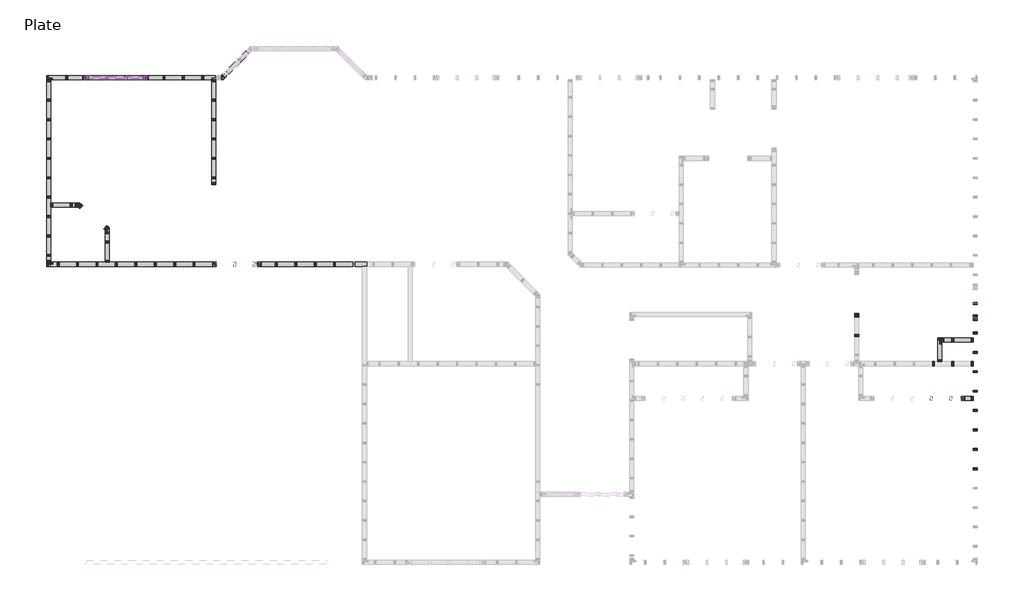
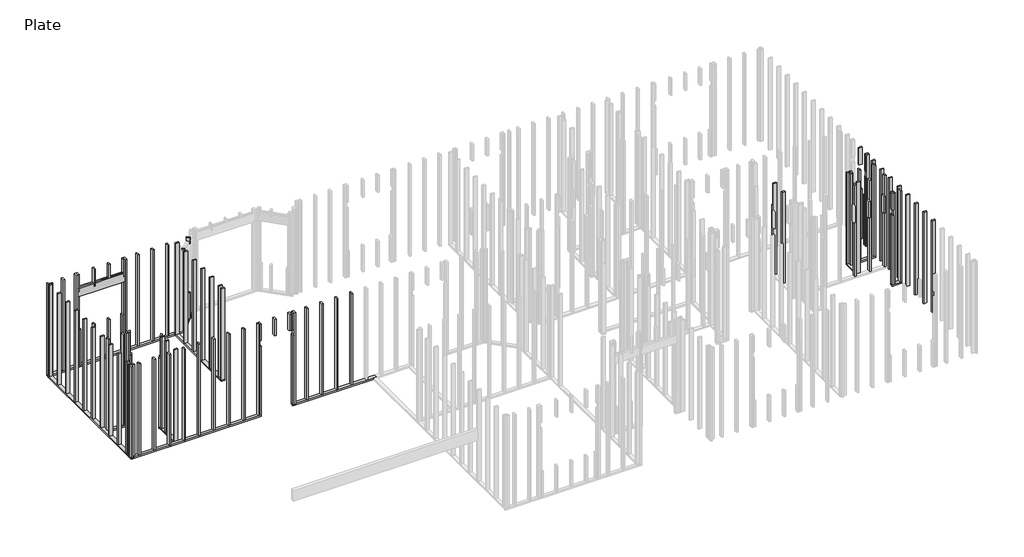
# One storey, part 3 of 5: 104 columns, 15 beams.
"""IFC4 building model written with IfcOpenShell, lengths in millimetres."""

import ifcopenshell
import ifcopenshell.guid

model = None  # the IFC model being written
_history = None  # IfcOwnerHistory: only IFC2X3 demands one
_inside = {}  # id of a spatial element -> (the spatial element, [elements in it])
_under = {}  # id of a project, library or spatial element -> (it, [spatial elements below it])
_declared = {}  # id of a project -> (the project, [libraries it declares])
_typed = {}  # id of a type object -> (the type object, [elements of that type])
_made_of = {}  # id of a material, layer set ... -> (it, [elements and type objects made of it])


def new_model(schema):
    """Start an empty IFC model of exactly this schema.

    Asked for "IFC4X3", IfcOpenShell would pick the latest addendum, in which some entities
    have other attributes; the version numbers below select the first issue.
    IFC2X3 requires an IfcOwnerHistory on every rooted entity: one is made here for all.
    """
    global model, _history
    if schema == "IFC4X3":
        model = ifcopenshell.file(schema_version=(4, 3, 0, 0))
    else:
        model = ifcopenshell.file(schema=schema)
    _inside.clear()
    _under.clear()
    _declared.clear()
    _typed.clear()
    _made_of.clear()
    _history = None
    if model.schema == "IFC2X3":
        org = make("IfcOrganization", Name="unknown")
        user = make(
            "IfcPersonAndOrganization",
            ThePerson=make("IfcPerson", FamilyName="unknown"),
            TheOrganization=org,
        )
        app = make(
            "IfcApplication",
            ApplicationDeveloper=org,
            Version="unknown",
            ApplicationFullName="unknown",
            ApplicationIdentifier="unknown",
        )
        _history = make(
            "IfcOwnerHistory",
            OwningUser=user,
            OwningApplication=app,
            ChangeAction="ADDED",
            CreationDate=0,
        )
    return model


def make(cls, **values):
    """One entity of the class cls with the attributes given. An attribute that is None is left unset."""
    return model.create_entity(
        cls, **{name: value for name, value in values.items() if value is not None}
    )


def rooted(cls, **values):
    """An entity with a GlobalId (a new one), such as an element, a storey or a relation."""
    return make(cls, GlobalId=ifcopenshell.guid.new(), OwnerHistory=_history, **values)


def si_unit(unit_type, name, prefix=None):
    """IfcSIUnit, for example si_unit("LENGTHUNIT", "METRE", prefix="MILLI")."""
    return make("IfcSIUnit", UnitType=unit_type, Prefix=prefix, Name=name)


def assignment(units):
    """IfcUnitAssignment: the units of a project."""
    return None if units is None else make("IfcUnitAssignment", Units=units)


def point(xyz):
    """IfcCartesianPoint."""
    return None if xyz is None else make("IfcCartesianPoint", Coordinates=xyz)


def direction(xyz):
    """IfcDirection."""
    return None if xyz is None else make("IfcDirection", DirectionRatios=xyz)


def frame(location, z_axis=None, x_axis=None):
    """IfcAxis2Placement3D, a coordinate frame: its origin and axes. An axis left out is left unset."""
    return make(
        "IfcAxis2Placement3D",
        Location=point(location),
        Axis=direction(z_axis),
        RefDirection=direction(x_axis),
    )


def origin():
    """The frame at (0, 0, 0) with its axes left unset."""
    return frame((0.0, 0.0, 0.0))


def place(relative_to, where):
    """IfcLocalPlacement: puts the frame where relative to a parent placement (None: the world)."""
    return make(
        "IfcLocalPlacement", PlacementRelTo=relative_to, RelativePlacement=where
    )


def context(
    kind, dimensions, precision=None, world=None, true_north=None, identifier=None
):
    """IfcGeometricRepresentationContext, for example the 3D "Model" context."""
    return make(
        "IfcGeometricRepresentationContext",
        ContextIdentifier=identifier,
        ContextType=kind,
        CoordinateSpaceDimension=dimensions,
        Precision=precision,
        WorldCoordinateSystem=world,
        TrueNorth=true_north,
    )


def project(units=None, contexts=None):
    """IfcProject with its units and contexts."""
    return rooted(
        "IfcProject",
        Name="project",
        RepresentationContexts=contexts,
        UnitsInContext=assignment(units),
    )


def spatial(cls, under=None, at=None, **own):
    """A site, building, storey or space (cls), placed at a placement, below another one or the project."""
    s = rooted(cls, ObjectPlacement=at, **own)
    if under is not None:
        _under.setdefault(under.id(), (under, []))[1].append(s)
    return s


def polyline(points):
    """IfcPolyline through the points."""
    return make("IfcPolyline", Points=[point(p) for p in points])


def outline(outer, holes=None, kind="AREA"):
    """IfcArbitraryClosedProfileDef: a profile drawn as a closed curve; with holes, ...WithVoids."""
    if holes is None:
        return make("IfcArbitraryClosedProfileDef", ProfileType=kind, OuterCurve=outer)
    return make(
        "IfcArbitraryProfileDefWithVoids",
        ProfileType=kind,
        OuterCurve=outer,
        InnerCurves=holes,
    )


def extrude(swept, where, along, depth):
    """IfcExtrudedAreaSolid: the profile swept, set in the frame where, extruded along a direction by depth."""
    return make(
        "IfcExtrudedAreaSolid",
        SweptArea=swept,
        Position=where,
        ExtrudedDirection=direction(along),
        Depth=depth,
    )


def shape(context_of_items, identifier, shape_type, items):
    """IfcShapeRepresentation: the items that make up one representation, for example the "Body"."""
    return make(
        "IfcShapeRepresentation",
        ContextOfItems=context_of_items,
        RepresentationIdentifier=identifier,
        RepresentationType=shape_type,
        Items=items,
    )


def source(mapping_origin, context_of_items, identifier, shape_type, items):
    """IfcRepresentationMap: a shape defined once, which mapped items show again and again."""
    return make(
        "IfcRepresentationMap",
        MappingOrigin=mapping_origin,
        MappedRepresentation=shape(context_of_items, identifier, shape_type, items),
    )


def transform(
    local_origin,
    x_axis=None,
    y_axis=None,
    z_axis=None,
    scale=None,
    scale2=None,
    scale3=None,
    uniform=True,
):
    """IfcCartesianTransformationOperator3D, or its non-uniform kind. x_axis, y_axis, z_axis: its Axis1, 2, 3."""
    if uniform:
        return make(
            "IfcCartesianTransformationOperator3D",
            Axis1=direction(x_axis),
            Axis2=direction(y_axis),
            LocalOrigin=point(local_origin),
            Scale=scale,
            Axis3=direction(z_axis),
        )
    return make(
        "IfcCartesianTransformationOperator3DnonUniform",
        Axis1=direction(x_axis),
        Axis2=direction(y_axis),
        LocalOrigin=point(local_origin),
        Scale=scale,
        Axis3=direction(z_axis),
        Scale2=scale2,
        Scale3=scale3,
    )


def mapped(mapping_source, mapping_target):
    """IfcMappedItem: shows the shape of a source again, moved by a transform."""
    return make(
        "IfcMappedItem", MappingSource=mapping_source, MappingTarget=mapping_target
    )


def made_of(thing, what):
    """Note that an element or type object is made of a material, layer set ...; save() writes the relation."""
    if what is not None:
        _made_of.setdefault(what.id(), (what, []))[1].append(thing)
    return thing


def element(
    cls,
    number,
    at=None,
    inside=None,
    cuts=None,
    type_object=None,
    material=None,
    context=None,
    identifier="Body",
    shape_type=None,
    held_by="IfcProductDefinitionShape",
    body=None,
    shapes=None,
    **own,
):
    """One element of the class cls, such as IfcWall. Its Tag is "e" and its number.

    at: its placement. inside: the storey or other place that contains it. cuts: it is an
    opening in that element (IfcRelVoidsElement). A single representation is given by context,
    identifier, shape_type and body (its items); several are given by shapes. held_by: the class
    of the entity that holds the representations. save() writes the other relations.
    """
    e = rooted(cls, Tag="e%d" % number, ObjectPlacement=at, **own)
    if body is not None:
        shapes = [shape(context, identifier, shape_type, body)]
    if shapes is not None:
        e.Representation = make(held_by, Representations=shapes)
    if inside is not None:
        _inside.setdefault(inside.id(), (inside, []))[1].append(e)
    if cuts is not None:
        rooted(
            "IfcRelVoidsElement", RelatingBuildingElement=cuts, RelatedOpeningElement=e
        )
    if type_object is not None:
        _typed.setdefault(type_object.id(), (type_object, []))[1].append(e)
    return made_of(e, material)


def aggregate(whole, parts):
    """IfcRelAggregates: a whole, such as a stair, and the parts it consists of."""
    return rooted("IfcRelAggregates", RelatingObject=whole, RelatedObjects=parts)


def save(model, path):
    """Write the relations noted so far, then the file.

    IfcRelAggregates (storeys below a building ...), IfcRelContainedInSpatialStructure (elements
    in a storey), IfcRelDefinesByType, IfcRelAssociatesMaterial and IfcRelDeclares: one each for
    every whole, place, type object, material and project.
    """
    for whole, parts in _under.values():
        aggregate(whole, parts)
    for where, things in _inside.values():
        rooted(
            "IfcRelContainedInSpatialStructure",
            RelatedElements=things,
            RelatingStructure=where,
        )
    for kind, things in _typed.values():
        rooted("IfcRelDefinesByType", RelatedObjects=things, RelatingType=kind)
    for what, things in _made_of.values():
        rooted("IfcRelAssociatesMaterial", RelatedObjects=things, RelatingMaterial=what)
    for by, libraries in _declared.values():
        rooted("IfcRelDeclares", RelatingContext=by, RelatedDefinitions=libraries)
    model.write(path)


def dimension_lumber_2x10_header_exterior_8d927054(model_context):
    return source(origin(), model_context, "Body", "SweptSolid", [
        extrude(outline(polyline([(468.709375, 19.05), (468.709375, -19.05), (-826.690625, -19.05), (-826.690625, 19.05), (468.709375, 19.05)])), frame((0.0, 0.0, -117.475), z_axis=(0.0, 0.0, 1.0), x_axis=(1.0, 0.0, 0.0)), (0.0, 0.0, 1.0), 234.95),
    ])


def dimension_lumber_supporting_bottom_plate_fd513b8e(model_context):
    return source(origin(), model_context, "Body", "SweptSolid", [
        extrude(outline(polyline([(1118.39375, 44.45), (1118.39375, -44.45), (-1165.225, -44.45), (-1165.225, 44.45), (1118.39375, 44.45)])), frame((0.0, 0.0, -19.05), z_axis=(0.0, 0.0, 1.0), x_axis=(1.0, 0.0, 0.0)), (0.0, 0.0, 1.0), 38.1),
    ])


def dimension_lumber_supporting_bottom_plate_14fdda6b(model_context):
    return source(origin(), model_context, "Body", "SweptSolid", [
        extrude(outline(polyline([(1910.55625, 44.45), (1910.55625, -44.45), (-1999.45625, -44.45), (-1999.45625, 44.45), (1910.55625, 44.45)])), frame((0.0, 0.0, -19.05), z_axis=(0.0, 0.0, 1.0), x_axis=(1.0, 0.0, 0.0)), (0.0, 0.0, 1.0), 38.1),
    ])


def dimension_lumber_supporting_bottom_plate_770482cb(model_context):
    return source(origin(), model_context, "Body", "SweptSolid", [
        extrude(outline(polyline([(1708.546875, 44.45), (1708.546875, -44.45), (-1752.996875, -44.45), (-1752.996875, 44.45), (1708.546875, 44.45)])), frame((0.0, 0.0, -19.05), z_axis=(0.0, 0.0, 1.0), x_axis=(1.0, 0.0, 0.0)), (0.0, 0.0, 1.0), 38.1),
    ])


def dimension_lumber_supporting_bottom_plate_d1710e57(model_context):
    return source(origin(), model_context, "Body", "SweptSolid", [
        extrude(outline(polyline([(1739.2219145, 44.45), (1739.2219145, -44.45), (-454.81875, -44.45), (-454.81875, 44.45), (1739.2219145, 44.45)])), frame((0.0, 0.0, -19.05), z_axis=(0.0, 0.0, 1.0), x_axis=(1.0, 0.0, 0.0)), (0.0, 0.0, 1.0), 38.1),
    ])


def dimension_lumber_supporting_bottom_plate_47a8c852(model_context):
    return source(origin(), model_context, "Body", "SweptSolid", [
        extrude(outline(polyline([(292.0, 44.45), (292.0, -44.45), (-203.1, -44.45), (-203.1, 44.45), (292.0, 44.45)])), frame((0.0, 0.0, -19.05), z_axis=(0.0, 0.0, 1.0), x_axis=(1.0, 0.0, 0.0)), (0.0, 0.0, 1.0), 38.1),
    ])


def dimension_lumber_supporting_bottom_plate_e3733361(model_context):
    return source(origin(), model_context, "Body", "SweptSolid", [
        extrude(outline(polyline([(328.9051334, 44.45), (328.9051334, -44.45), (-328.9051334, -44.45), (-328.9051334, 44.45), (328.9051334, 44.45)])), frame((0.0, 0.0, -19.05), z_axis=(0.0, 0.0, 1.0), x_axis=(1.0, 0.0, 0.0)), (0.0, 0.0, 1.0), 38.1),
    ])


def dimension_lumber_supporting_bottom_plate_76e17ce6(model_context):
    return source(origin(), model_context, "Body", "SweptSolid", [
        extrude(outline(polyline([(146.8437503, 44.45), (146.8437503, -44.45), (-102.3937503, -44.45), (-102.3937503, 44.45), (146.8437503, 44.45)])), frame((0.0, 0.0, -19.05), z_axis=(0.0, 0.0, 1.0), x_axis=(1.0, 0.0, 0.0)), (0.0, 0.0, 1.0), 38.1),
    ])


def dimension_lumber_column_2x4_07183c39(model_context):
    return source(origin(), model_context, "Body", "SweptSolid", [
        extrude(outline(polyline([(19.05, 44.45), (19.05, -44.45), (-19.05, -44.45), (-19.05, 44.45), (19.05, 44.45)])), frame((0.0, 0.0, 56.35625), z_axis=(0.0, 0.0, 1.0), x_axis=(1.0, 0.0, 0.0)), (0.0, 0.0, 1.0), 2636.04375),
    ])


def dimension_lumber_column_2x4_f24b5bbb(model_context):
    return source(origin(), model_context, "Body", "SweptSolid", [
        extrude(outline(polyline([(19.05, -44.45), (-19.05, -44.45), (-19.05, 44.45), (19.05, 44.45), (19.05, -44.45)])), frame((0.0, 0.0, 56.35625), z_axis=(0.0, 0.0, 1.0), x_axis=(1.0, 0.0, 0.0)), (0.0, 0.0, 1.0), 2636.04375),
    ])


def dimension_lumber_column_2x4_1c0ee4a5(model_context):
    return source(origin(), model_context, "Body", "SweptSolid", [
        extrude(outline(polyline([(19.05, -44.45), (-19.05, -44.45), (-19.05, 44.45), (19.05, 44.45), (19.05, -44.45)])), frame((0.0, 0.0, 56.35625), z_axis=(0.0, 0.0, 1.0), x_axis=(1.0, 0.0, 0.0)), (0.0, 0.0, 1.0), 2331.24375),
    ])


def dimension_lumber_column_2x4_0f816ddf(model_context):
    return source(origin(), model_context, "Body", "SweptSolid", [
        extrude(outline(polyline([(19.05, 44.45), (19.05, -44.45), (-19.05, -44.45), (-19.05, 44.45), (19.05, 44.45)])), frame((0.0, 0.0, 56.35625), z_axis=(0.0, 0.0, 1.0), x_axis=(1.0, 0.0, 0.0)), (0.0, 0.0, 1.0), 1999.853125),
    ])


def dimension_lumber_column_2x4_c2f848da(model_context):
    return source(origin(), model_context, "Body", "SweptSolid", [
        extrude(outline(polyline([(19.05, 44.45), (19.05, -44.45), (-19.05, -44.45), (-19.05, 44.45), (19.05, 44.45)])), frame((0.0, 0.0, 2208.609375), z_axis=(0.0, 0.0, 1.0), x_axis=(1.0, 0.0, 0.0)), (0.0, 0.0, 1.0), 483.790625),
    ])


def dimension_lumber_column_2x4_1a929157(model_context):
    return source(origin(), model_context, "Body", "SweptSolid", [
        extrude(outline(polyline([(19.05, 44.45), (19.05, -44.45), (-19.05, -44.45), (-19.05, 44.45), (19.05, 44.45)])), frame((0.0, 0.0, 2208.609375), z_axis=(0.0, 0.0, 1.0), x_axis=(1.0, 0.0, 0.0)), (0.0, 0.0, 1.0), 178.990625),
    ])


def dimension_lumber_column_2x4_35883525(model_context):
    return source(origin(), model_context, "Body", "SweptSolid", [
        extrude(outline(polyline([(19.05, 44.45), (19.05, -44.45), (-19.05, -44.45), (-19.05, 44.45), (19.05, 44.45)])), frame((0.0, 0.0, 56.35625), z_axis=(0.0, 0.0, 1.0), x_axis=(1.0, 0.0, 0.0)), (0.0, 0.0, 1.0), 742.553125),
    ])


def dimension_lumber_column_2x4_e2d4624f(model_context):
    return source(origin(), model_context, "Body", "SweptSolid", [
        extrude(outline(polyline([(19.05, 44.45), (19.05, -44.45), (-19.05, -44.45), (-19.05, 44.45), (19.05, 44.45)])), frame((0.0, 0.0, 56.35625), z_axis=(0.0, 0.0, 1.0), x_axis=(1.0, 0.0, 0.0)), (0.0, 0.0, 1.0), 1047.353125),
    ])


def dimension_lumber_column_2x4_c4e013fe(model_context):
    return source(origin(), model_context, "Body", "SweptSolid", [
        extrude(outline(polyline([(19.05, 44.45), (19.05, -44.45), (-19.05, -44.45), (-19.05, 44.45), (19.05, 44.45)])), frame((0.0, 0.0, 56.35625), z_axis=(0.0, 0.0, 1.0), x_axis=(1.0, 0.0, 0.0)), (0.0, 0.0, 1.0), 1444.228125),
    ])


model = new_model("IFC4")

# Units and contexts
model_context = context("Model", 3, world=origin())
ifc_project = project(units=[si_unit("LENGTHUNIT", "METRE", prefix="MILLI")], contexts=[model_context])

# Site, building, storey
site = spatial("IfcSite", under=ifc_project)
building = spatial("IfcBuilding", under=site)
storey = spatial("IfcBuildingStorey", under=building, Name="Plate", Elevation=56.35625)

# Beams
placement = place(None, origin())
dimension_lumber_2x10_header_exterior_shape = dimension_lumber_2x10_header_exterior_8d927054(model_context)
element("IfcBeam", 1, ObjectType="Dimension Lumber : 2x10 Header Exterior", at=placement, inside=storey, context=model_context, shape_type="MappedRepresentation", body=[
    mapped(dimension_lumber_2x10_header_exterior_shape, transform((-4972.0933507, 4418.3834053, 2173.684375), x_axis=(-1.0, 0.0, 0.0), y_axis=(0.0, -1.0, 0.0), z_axis=(0.0, 0.0, 1.0))),
])
element("IfcBeam", 2, ObjectType="Dimension Lumber : 2x10 Header Exterior", at=placement, inside=storey, context=model_context, shape_type="MappedRepresentation", body=[
    mapped(dimension_lumber_2x10_header_exterior_shape, transform((-4972.0933507, 4469.1834053, 2173.684375), x_axis=(-1.0, 0.0, 0.0), y_axis=(0.0, -1.0, 0.0), z_axis=(0.0, 0.0, 1.0))),
])
element("IfcBeam", 3, ObjectType="Dimension Lumber : Supporting Bottom Plate", at=placement, inside=storey, context=model_context, shape_type="SweptSolid", body=[
    extrude(outline(polyline([(-2583.3027251, 4488.2334053), (-2546.4791394, 4399.3334053), (-6240.9027251, 4399.3334053), (-6240.9027251, 4488.2334053), (-2583.3027251, 4488.2334053)])), frame((0.0, 0.0, 18.25625), z_axis=(0.0, 0.0, 1.0), x_axis=(1.0, 0.0, 0.0)), (0.0, 0.0, 1.0), 38.1),
])
element("IfcBeam", 4, ObjectType="Dimension Lumber : Supporting Bottom Plate", at=placement, inside=storey, context=model_context, shape_type="SweptSolid", body=[
    extrude(outline(polyline([(-1973.7027251, 5097.8334053), (-1936.8791394, 5008.9334053), (-2546.4791394, 4399.3334053), (-2583.3027251, 4488.2334053), (-1973.7027251, 5097.8334053)])), frame((0.0, 0.0, 18.25625), z_axis=(0.0, 0.0, 1.0), x_axis=(1.0, 0.0, 0.0)), (0.0, 0.0, 1.0), 38.1),
])
element("IfcBeam", 5, ObjectType="Dimension Lumber : Supporting Bottom Plate", at=placement, inside=storey, context=model_context, shape_type="SweptSolid", body=[
    extrude(outline(polyline([(-5544.0627459, 1818.4935621), (-5576.4196998, 1729.5935621), (-6152.0027251, 1729.5935621), (-6152.0027251, 1818.4935621), (-5544.0627459, 1818.4935621)])), frame((0.0, 0.0, 18.25625), z_axis=(0.0, 0.0, 1.0), x_axis=(1.0, 0.0, 0.0)), (0.0, 0.0, 1.0), 38.1),
])
element("IfcBeam", 6, ObjectType="Dimension Lumber : Supporting Bottom Plate", at=placement, inside=storey, context=model_context, shape_type="SweptSolid", body=[
    extrude(outline(polyline([(-5485.6901594, 1769.5131462), (-5542.8339779, 1701.4117952), (-5576.4196998, 1729.5935621), (-5544.0627459, 1818.4935621), (-5485.6901594, 1769.5131462)])), frame((0.0, 0.0, 18.25625), z_axis=(0.0, 0.0, 1.0), x_axis=(1.0, 0.0, 0.0)), (0.0, 0.0, 1.0), 38.1),
])
element("IfcBeam", 7, ObjectType="Dimension Lumber : Supporting Bottom Plate", at=placement, inside=storey, context=model_context, shape_type="SweptSolid", body=[
    extrude(outline(polyline([(-5012.1263621, 1256.0952306), (-4923.2263621, 1297.5499814), (-4923.2263621, 578.2209053), (-5012.1263621, 578.2209053), (-5012.1263621, 1256.0952306)])), frame((0.0, 0.0, 18.25625), z_axis=(0.0, 0.0, 1.0), x_axis=(1.0, 0.0, 0.0)), (0.0, 0.0, 1.0), 38.1),
])
element("IfcBeam", 8, ObjectType="Dimension Lumber : Supporting Bottom Plate", at=placement, inside=storey, context=model_context, shape_type="SweptSolid", body=[
    extrude(outline(polyline([(-4923.2263621, 1297.5499814), (-5012.1263621, 1256.0952306), (-5038.762371, 1278.4454958), (-4981.6185525, 1346.5468468), (-4923.2263621, 1297.5499814)])), frame((0.0, 0.0, 18.25625), z_axis=(0.0, 0.0, 1.0), x_axis=(1.0, 0.0, 0.0)), (0.0, 0.0, 1.0), 38.1),
])
dimension_lumber_supporting_bottom_plate_shape = dimension_lumber_supporting_bottom_plate_fd513b8e(model_context)
element("IfcBeam", 9, ObjectType="Dimension Lumber : Supporting Bottom Plate", at=placement, inside=storey, context=model_context, shape_type="MappedRepresentation", body=[
    mapped(dimension_lumber_supporting_bottom_plate_shape, transform((-708.4652251, 533.7709053, 37.30625), x_axis=(-1.0, 0.0, 0.0), y_axis=(0.0, -1.0, 0.0), z_axis=(0.0, 0.0, 1.0))),
])
dimension_lumber_supporting_bottom_plate_2_shape = dimension_lumber_supporting_bottom_plate_14fdda6b(model_context)
element("IfcBeam", 10, ObjectType="Dimension Lumber : Supporting Bottom Plate", at=placement, inside=storey, context=model_context, shape_type="MappedRepresentation", body=[
    mapped(dimension_lumber_supporting_bottom_plate_2_shape, transform((-6196.4527251, 2488.7771553, 37.30625), x_axis=(0.0, 1.0, 0.0), y_axis=(-1.0, 0.0, 0.0), z_axis=(0.0, 0.0, 1.0))),
])
dimension_lumber_supporting_bottom_plate_3_shape = dimension_lumber_supporting_bottom_plate_770482cb(model_context)
element("IfcBeam", 11, ObjectType="Dimension Lumber : Supporting Bottom Plate", at=placement, inside=storey, context=model_context, shape_type="MappedRepresentation", body=[
    mapped(dimension_lumber_supporting_bottom_plate_3_shape, transform((-4443.4558501, 533.7709053, 37.30625), x_axis=(-1.0, 0.0, 0.0), y_axis=(0.0, -1.0, 0.0), z_axis=(0.0, 0.0, 1.0))),
])
dimension_lumber_supporting_bottom_plate_4_shape = dimension_lumber_supporting_bottom_plate_d1710e57(model_context)
element("IfcBeam", 12, ObjectType="Dimension Lumber : Supporting Bottom Plate", at=placement, inside=storey, context=model_context, shape_type="MappedRepresentation", body=[
    mapped(dimension_lumber_supporting_bottom_plate_4_shape, transform((-2742.0527251, 3944.5146553, 37.30625), x_axis=(0.0, -1.0, 0.0), y_axis=(1.0, 0.0, 0.0), z_axis=(0.0, 0.0, 1.0))),
])
dimension_lumber_supporting_bottom_plate_5_shape = dimension_lumber_supporting_bottom_plate_47a8c852(model_context)
element("IfcBeam", 13, ObjectType="Dimension Lumber : Supporting Bottom Plate", at=placement, inside=storey, context=model_context, shape_type="MappedRepresentation", body=[
    mapped(dimension_lumber_supporting_bottom_plate_5_shape, transform((12452.9120082, -1298.3040947, 37.30625), x_axis=(0.0, 1.0, 0.0), y_axis=(-1.0, 0.0, 0.0), z_axis=(0.0, 0.0, 1.0))),
])
dimension_lumber_supporting_bottom_plate_6_shape = dimension_lumber_supporting_bottom_plate_e3733361(model_context)
element("IfcBeam", 14, ObjectType="Dimension Lumber : Supporting Bottom Plate", at=placement, inside=storey, context=model_context, shape_type="MappedRepresentation", body=[
    mapped(dimension_lumber_supporting_bottom_plate_6_shape, transform((12826.2671415, -1050.7540947, 37.30625), x_axis=(1.0, 0.0, 0.0), y_axis=(0.0, 1.0, 0.0), z_axis=(0.0, 0.0, 1.0))),
])
dimension_lumber_supporting_bottom_plate_7_shape = dimension_lumber_supporting_bottom_plate_76e17ce6(model_context)
element("IfcBeam", 15, ObjectType="Dimension Lumber : Supporting Bottom Plate", at=placement, inside=storey, context=model_context, shape_type="MappedRepresentation", body=[
    mapped(dimension_lumber_supporting_bottom_plate_7_shape, transform((13052.7785246, -2276.1040947, 37.30625), x_axis=(-1.0, 0.0, 0.0), y_axis=(0.0, -1.0, 0.0), z_axis=(0.0, 0.0, 1.0))),
])

# Columns
dimension_lumber_column_2x4_shape = dimension_lumber_column_2x4_07183c39(model_context)
element("IfcColumn", 16, ObjectType="Dimension Lumber-Column : 2x4", at=placement, inside=storey, context=model_context, shape_type="MappedRepresentation", body=[
    mapped(dimension_lumber_column_2x4_shape, transform((13199.6222749, -625.1040947, 0.0), x_axis=(0.0, 1.0, 0.0), y_axis=(-1.0, 0.0, 0.0), z_axis=(0.0, 0.0, 1.0))),
])
element("IfcColumn", 17, ObjectType="Dimension Lumber-Column : 2x4", at=placement, inside=storey, context=model_context, shape_type="MappedRepresentation", body=[
    mapped(dimension_lumber_column_2x4_shape, transform((13199.6222749, -902.9165947, 0.0), x_axis=(0.0, 1.0, 0.0), y_axis=(-1.0, 0.0, 0.0), z_axis=(0.0, 0.0, 1.0))),
])
element("IfcColumn", 18, ObjectType="Dimension Lumber-Column : 2x4", at=placement, inside=storey, context=model_context, shape_type="MappedRepresentation", body=[
    mapped(dimension_lumber_column_2x4_shape, transform((13199.6222749, -1309.3165947, 0.0), x_axis=(0.0, 1.0, 0.0), y_axis=(-1.0, 0.0, 0.0), z_axis=(0.0, 0.0, 1.0))),
])
element("IfcColumn", 19, ObjectType="Dimension Lumber-Column : 2x4", at=placement, inside=storey, context=model_context, shape_type="MappedRepresentation", body=[
    mapped(dimension_lumber_column_2x4_shape, transform((13199.6222749, -1715.7165947, 0.0), x_axis=(0.0, 1.0, 0.0), y_axis=(-1.0, 0.0, 0.0), z_axis=(0.0, 0.0, 1.0))),
])
element("IfcColumn", 20, ObjectType="Dimension Lumber-Column : 2x4", at=placement, inside=storey, context=model_context, shape_type="MappedRepresentation", body=[
    mapped(dimension_lumber_column_2x4_shape, transform((13199.6222749, -2122.1165947, 0.0), x_axis=(0.0, 1.0, 0.0), y_axis=(-1.0, 0.0, 0.0), z_axis=(0.0, 0.0, 1.0))),
])
element("IfcColumn", 21, ObjectType="Dimension Lumber-Column : 2x4", at=placement, inside=storey, context=model_context, shape_type="MappedRepresentation", body=[
    mapped(dimension_lumber_column_2x4_shape, transform((13199.6222749, -2528.5165947, 0.0), x_axis=(0.0, 1.0, 0.0), y_axis=(-1.0, 0.0, 0.0), z_axis=(0.0, 0.0, 1.0))),
])
element("IfcColumn", 22, ObjectType="Dimension Lumber-Column : 2x4", at=placement, inside=storey, context=model_context, shape_type="MappedRepresentation", body=[
    mapped(dimension_lumber_column_2x4_shape, transform((13199.6222749, -2934.9165947, 0.0), x_axis=(0.0, 1.0, 0.0), y_axis=(-1.0, 0.0, 0.0), z_axis=(0.0, 0.0, 1.0))),
])
element("IfcColumn", 23, ObjectType="Dimension Lumber-Column : 2x4", at=placement, inside=storey, context=model_context, shape_type="MappedRepresentation", body=[
    mapped(dimension_lumber_column_2x4_shape, transform((13199.6222749, -3341.3165947, 0.0), x_axis=(0.0, 1.0, 0.0), y_axis=(-1.0, 0.0, 0.0), z_axis=(0.0, 0.0, 1.0))),
])
element("IfcColumn", 24, ObjectType="Dimension Lumber-Column : 2x4", at=placement, inside=storey, context=model_context, shape_type="MappedRepresentation", body=[
    mapped(dimension_lumber_column_2x4_shape, transform((13199.6222749, -3747.7165947, 0.0), x_axis=(0.0, 1.0, 0.0), y_axis=(-1.0, 0.0, 0.0), z_axis=(0.0, 0.0, 1.0))),
])
element("IfcColumn", 25, ObjectType="Dimension Lumber-Column : 2x4", at=placement, inside=storey, context=model_context, shape_type="MappedRepresentation", body=[
    mapped(dimension_lumber_column_2x4_shape, transform((13136.1222749, -1545.8540947, 0.0), x_axis=(1.0, 0.0, 0.0), y_axis=(0.0, 1.0, 0.0), z_axis=(0.0, 0.0, 1.0))),
])
element("IfcColumn", 26, ObjectType="Dimension Lumber-Column : 2x4", at=placement, inside=storey, context=model_context, shape_type="MappedRepresentation", body=[
    mapped(dimension_lumber_column_2x4_shape, transform((12729.7222749, -1545.8540947, 0.0), x_axis=(1.0, 0.0, 0.0), y_axis=(0.0, 1.0, 0.0), z_axis=(0.0, 0.0, 1.0))),
])
element("IfcColumn", 27, ObjectType="Dimension Lumber-Column : 2x4", at=placement, inside=storey, context=model_context, shape_type="MappedRepresentation", body=[
    mapped(dimension_lumber_column_2x4_shape, transform((12323.3222749, -1545.8540947, 0.0), x_axis=(1.0, 0.0, 0.0), y_axis=(0.0, 1.0, 0.0), z_axis=(0.0, 0.0, 1.0))),
])
element("IfcColumn", 28, ObjectType="Dimension Lumber-Column : 2x4", at=placement, inside=storey, context=model_context, shape_type="MappedRepresentation", body=[
    mapped(dimension_lumber_column_2x4_shape, transform((-2742.0527251, 4380.2834053, 0.0), x_axis=(0.0, -1.0, 0.0), y_axis=(1.0, 0.0, 0.0), z_axis=(0.0, 0.0, 1.0))),
])
element("IfcColumn", 29, ObjectType="Dimension Lumber-Column : 2x4", at=placement, inside=storey, context=model_context, shape_type="MappedRepresentation", body=[
    mapped(dimension_lumber_column_2x4_shape, transform((-2742.0527251, 3973.8834053, 0.0), x_axis=(0.0, -1.0, 0.0), y_axis=(1.0, 0.0, 0.0), z_axis=(0.0, 0.0, 1.0))),
])
element("IfcColumn", 30, ObjectType="Dimension Lumber-Column : 2x4", at=placement, inside=storey, context=model_context, shape_type="MappedRepresentation", body=[
    mapped(dimension_lumber_column_2x4_shape, transform((-2742.0527251, 3567.4834053, 0.0), x_axis=(0.0, -1.0, 0.0), y_axis=(1.0, 0.0, 0.0), z_axis=(0.0, 0.0, 1.0))),
])
element("IfcColumn", 31, ObjectType="Dimension Lumber-Column : 2x4", at=placement, inside=storey, context=model_context, shape_type="MappedRepresentation", body=[
    mapped(dimension_lumber_column_2x4_shape, transform((-2742.0527251, 3161.0834053, 0.0), x_axis=(0.0, -1.0, 0.0), y_axis=(1.0, 0.0, 0.0), z_axis=(0.0, 0.0, 1.0))),
])
element("IfcColumn", 32, ObjectType="Dimension Lumber-Column : 2x4", at=placement, inside=storey, context=model_context, shape_type="MappedRepresentation", body=[
    mapped(dimension_lumber_column_2x4_shape, transform((-2742.0527251, 2754.6834053, 0.0), x_axis=(0.0, -1.0, 0.0), y_axis=(1.0, 0.0, 0.0), z_axis=(0.0, 0.0, 1.0))),
])
element("IfcColumn", 33, ObjectType="Dimension Lumber-Column : 2x4", at=placement, inside=storey, context=model_context, shape_type="MappedRepresentation", body=[
    mapped(dimension_lumber_column_2x4_shape, transform((-2742.0527251, 2348.2834053, 0.0), x_axis=(0.0, -1.0, 0.0), y_axis=(1.0, 0.0, 0.0), z_axis=(0.0, 0.0, 1.0))),
])
element("IfcColumn", 34, ObjectType="Dimension Lumber-Column : 2x4", at=placement, inside=storey, context=model_context, shape_type="MappedRepresentation", body=[
    mapped(dimension_lumber_column_2x4_shape, transform((-2742.0527251, 2224.3427408, 0.0), x_axis=(0.0, -1.0, 0.0), y_axis=(1.0, 0.0, 0.0), z_axis=(0.0, 0.0, 1.0))),
])
element("IfcColumn", 35, ObjectType="Dimension Lumber-Column : 2x4", at=placement, inside=storey, context=model_context, shape_type="MappedRepresentation", body=[
    mapped(dimension_lumber_column_2x4_shape, transform((10715.1847749, -547.7134697, 0.0), x_axis=(0.0, 1.0, 0.0), y_axis=(-1.0, 0.0, 0.0), z_axis=(0.0, 0.0, 1.0))),
])
element("IfcColumn", 36, ObjectType="Dimension Lumber-Column : 2x4", at=placement, inside=storey, context=model_context, shape_type="MappedRepresentation", body=[
    mapped(dimension_lumber_column_2x4_shape, transform((-211.9746001, 533.7709053, 0.0), x_axis=(1.0, 0.0, 0.0), y_axis=(0.0, 1.0, 0.0), z_axis=(0.0, 0.0, 1.0))),
])
element("IfcColumn", 37, ObjectType="Dimension Lumber-Column : 2x4", at=placement, inside=storey, context=model_context, shape_type="MappedRepresentation", body=[
    mapped(dimension_lumber_column_2x4_shape, transform((-618.3746001, 533.7709053, 0.0), x_axis=(1.0, 0.0, 0.0), y_axis=(0.0, 1.0, 0.0), z_axis=(0.0, 0.0, 1.0))),
])
element("IfcColumn", 38, ObjectType="Dimension Lumber-Column : 2x4", at=placement, inside=storey, context=model_context, shape_type="MappedRepresentation", body=[
    mapped(dimension_lumber_column_2x4_shape, transform((-1024.7746001, 533.7709053, 0.0), x_axis=(1.0, 0.0, 0.0), y_axis=(0.0, 1.0, 0.0), z_axis=(0.0, 0.0, 1.0))),
])
element("IfcColumn", 39, ObjectType="Dimension Lumber-Column : 2x4", at=placement, inside=storey, context=model_context, shape_type="MappedRepresentation", body=[
    mapped(dimension_lumber_column_2x4_shape, transform((-1431.1746001, 533.7709053, 0.0), x_axis=(1.0, 0.0, 0.0), y_axis=(0.0, 1.0, 0.0), z_axis=(0.0, 0.0, 1.0))),
])
element("IfcColumn", 40, ObjectType="Dimension Lumber-Column : 2x4", at=placement, inside=storey, context=model_context, shape_type="MappedRepresentation", body=[
    mapped(dimension_lumber_column_2x4_shape, transform((-1769.7089751, 533.7709053, 0.0), x_axis=(1.0, 0.0, 0.0), y_axis=(0.0, 1.0, 0.0), z_axis=(0.0, 0.0, 1.0))),
])
element("IfcColumn", 41, ObjectType="Dimension Lumber-Column : 2x4", at=placement, inside=storey, context=model_context, shape_type="MappedRepresentation", body=[
    mapped(dimension_lumber_column_2x4_shape, transform((-2747.6089751, 533.7709053, 0.0), x_axis=(1.0, 0.0, 0.0), y_axis=(0.0, 1.0, 0.0), z_axis=(0.0, 0.0, 1.0))),
])
element("IfcColumn", 42, ObjectType="Dimension Lumber-Column : 2x4", at=placement, inside=storey, context=model_context, shape_type="MappedRepresentation", body=[
    mapped(dimension_lumber_column_2x4_shape, transform((-3154.0089751, 533.7709053, 0.0), x_axis=(1.0, 0.0, 0.0), y_axis=(0.0, 1.0, 0.0), z_axis=(0.0, 0.0, 1.0))),
])
element("IfcColumn", 43, ObjectType="Dimension Lumber-Column : 2x4", at=placement, inside=storey, context=model_context, shape_type="MappedRepresentation", body=[
    mapped(dimension_lumber_column_2x4_shape, transform((-3560.4089751, 533.7709053, 0.0), x_axis=(1.0, 0.0, 0.0), y_axis=(0.0, 1.0, 0.0), z_axis=(0.0, 0.0, 1.0))),
])
element("IfcColumn", 44, ObjectType="Dimension Lumber-Column : 2x4", at=placement, inside=storey, context=model_context, shape_type="MappedRepresentation", body=[
    mapped(dimension_lumber_column_2x4_shape, transform((-3966.8089751, 533.7709053, 0.0), x_axis=(1.0, 0.0, 0.0), y_axis=(0.0, 1.0, 0.0), z_axis=(0.0, 0.0, 1.0))),
])
element("IfcColumn", 45, ObjectType="Dimension Lumber-Column : 2x4", at=placement, inside=storey, context=model_context, shape_type="MappedRepresentation", body=[
    mapped(dimension_lumber_column_2x4_shape, transform((-4373.2089751, 533.7709053, 0.0), x_axis=(1.0, 0.0, 0.0), y_axis=(0.0, 1.0, 0.0), z_axis=(0.0, 0.0, 1.0))),
])
element("IfcColumn", 46, ObjectType="Dimension Lumber-Column : 2x4", at=placement, inside=storey, context=model_context, shape_type="MappedRepresentation", body=[
    mapped(dimension_lumber_column_2x4_shape, transform((-4779.6089751, 533.7709053, 0.0), x_axis=(1.0, 0.0, 0.0), y_axis=(0.0, 1.0, 0.0), z_axis=(0.0, 0.0, 1.0))),
])
element("IfcColumn", 47, ObjectType="Dimension Lumber-Column : 2x4", at=placement, inside=storey, context=model_context, shape_type="MappedRepresentation", body=[
    mapped(dimension_lumber_column_2x4_shape, transform((-5186.0089751, 533.7709053, 0.0), x_axis=(1.0, 0.0, 0.0), y_axis=(0.0, 1.0, 0.0), z_axis=(0.0, 0.0, 1.0))),
])
element("IfcColumn", 48, ObjectType="Dimension Lumber-Column : 2x4", at=placement, inside=storey, context=model_context, shape_type="MappedRepresentation", body=[
    mapped(dimension_lumber_column_2x4_shape, transform((-5592.4089751, 533.7709053, 0.0), x_axis=(1.0, 0.0, 0.0), y_axis=(0.0, 1.0, 0.0), z_axis=(0.0, 0.0, 1.0))),
])
element("IfcColumn", 49, ObjectType="Dimension Lumber-Column : 2x4", at=placement, inside=storey, context=model_context, shape_type="MappedRepresentation", body=[
    mapped(dimension_lumber_column_2x4_shape, transform((-5998.8089751, 533.7709053, 0.0), x_axis=(1.0, 0.0, 0.0), y_axis=(0.0, 1.0, 0.0), z_axis=(0.0, 0.0, 1.0))),
])
element("IfcColumn", 50, ObjectType="Dimension Lumber-Column : 2x4", at=placement, inside=storey, context=model_context, shape_type="MappedRepresentation", body=[
    mapped(dimension_lumber_column_2x4_shape, transform((-6221.8527251, 533.7709053, 0.0), x_axis=(1.0, 0.0, 0.0), y_axis=(0.0, 1.0, 0.0), z_axis=(0.0, 0.0, 1.0))),
])
element("IfcColumn", 51, ObjectType="Dimension Lumber-Column : 2x4", at=placement, inside=storey, context=model_context, shape_type="MappedRepresentation", body=[
    mapped(dimension_lumber_column_2x4_shape, transform((-5726.5527251, 1774.0435621, 0.0), x_axis=(1.0, 0.0, 0.0), y_axis=(0.0, 1.0, 0.0), z_axis=(0.0, 0.0, 1.0))),
])
element("IfcColumn", 52, ObjectType="Dimension Lumber-Column : 2x4", at=placement, inside=storey, context=model_context, shape_type="MappedRepresentation", body=[
    mapped(dimension_lumber_column_2x4_shape, transform((-6132.9527251, 1774.0435621, 0.0), x_axis=(1.0, 0.0, 0.0), y_axis=(0.0, 1.0, 0.0), z_axis=(0.0, 0.0, 1.0))),
])
element("IfcColumn", 53, ObjectType="Dimension Lumber-Column : 2x4", at=placement, inside=storey, context=model_context, shape_type="MappedRepresentation", body=[
    mapped(dimension_lumber_column_2x4_shape, transform((-5558.0415085, 1772.1977826, 0.0), x_axis=(0.7660444431189741, -0.642787609686544, 0.0), y_axis=(0.642787609686544, 0.7660444431189741, 0.0), z_axis=(0.0, 0.0, 1.0))),
])
element("IfcColumn", 54, ObjectType="Dimension Lumber-Column : 2x4", at=placement, inside=storey, context=model_context, shape_type="MappedRepresentation", body=[
    mapped(dimension_lumber_column_2x4_shape, transform((-5620.2565644, 1774.0435621, 0.0), x_axis=(1.0, 0.0, 0.0), y_axis=(0.0, 1.0, 0.0), z_axis=(0.0, 0.0, 1.0))),
])
element("IfcColumn", 55, ObjectType="Dimension Lumber-Column : 2x4", at=placement, inside=storey, context=model_context, shape_type="MappedRepresentation", body=[
    mapped(dimension_lumber_column_2x4_shape, transform((-4966.391418, 1275.7444099, 0.0), x_axis=(0.7660444431189741, -0.642787609686544, 0.0), y_axis=(0.642787609686544, 0.7660444431189741, 0.0), z_axis=(0.0, 0.0, 1.0))),
])
element("IfcColumn", 56, ObjectType="Dimension Lumber-Column : 2x4", at=placement, inside=storey, context=model_context, shape_type="MappedRepresentation", body=[
    mapped(dimension_lumber_column_2x4_shape, transform((-5459.8527257, 4443.7834053, 0.0), x_axis=(1.0, 0.0, 0.0), y_axis=(0.0, 1.0, 0.0), z_axis=(0.0, 0.0, 1.0))),
])
element("IfcColumn", 57, ObjectType="Dimension Lumber-Column : 2x4", at=placement, inside=storey, context=model_context, shape_type="MappedRepresentation", body=[
    mapped(dimension_lumber_column_2x4_shape, transform((-4126.3527257, 4443.7834053, 0.0), x_axis=(1.0, 0.0, 0.0), y_axis=(0.0, 1.0, 0.0), z_axis=(0.0, 0.0, 1.0))),
])
element("IfcColumn", 58, ObjectType="Dimension Lumber-Column : 2x4", at=placement, inside=storey, context=model_context, shape_type="MappedRepresentation", body=[
    mapped(dimension_lumber_column_2x4_shape, transform((13136.1222749, -1050.7540947, 0.0), x_axis=(1.0, 0.0, 0.0), y_axis=(0.0, 1.0, 0.0), z_axis=(0.0, 0.0, 1.0))),
])
element("IfcColumn", 59, ObjectType="Dimension Lumber-Column : 2x4", at=placement, inside=storey, context=model_context, shape_type="MappedRepresentation", body=[
    mapped(dimension_lumber_column_2x4_shape, transform((12729.7222749, -1050.7540947, 0.0), x_axis=(1.0, 0.0, 0.0), y_axis=(0.0, 1.0, 0.0), z_axis=(0.0, 0.0, 1.0))),
])
element("IfcColumn", 60, ObjectType="Dimension Lumber-Column : 2x4", at=placement, inside=storey, context=model_context, shape_type="MappedRepresentation", body=[
    mapped(dimension_lumber_column_2x4_shape, transform((12516.4120082, -1050.7540947, 0.0), x_axis=(1.0, 0.0, 0.0), y_axis=(0.0, 1.0, 0.0), z_axis=(0.0, 0.0, 1.0))),
])
element("IfcColumn", 61, ObjectType="Dimension Lumber-Column : 2x4", at=placement, inside=storey, context=model_context, shape_type="MappedRepresentation", body=[
    mapped(dimension_lumber_column_2x4_shape, transform((12452.9120082, -1482.3540947, 0.0), x_axis=(0.0, 1.0, 0.0), y_axis=(-1.0, 0.0, 0.0), z_axis=(0.0, 0.0, 1.0))),
])
element("IfcColumn", 62, ObjectType="Dimension Lumber-Column : 2x4", at=placement, inside=storey, context=model_context, shape_type="MappedRepresentation", body=[
    mapped(dimension_lumber_column_2x4_shape, transform((12452.9120082, -1025.3540947, 0.0), x_axis=(0.0, 1.0, 0.0), y_axis=(-1.0, 0.0, 0.0), z_axis=(0.0, 0.0, 1.0))),
])
element("IfcColumn", 63, ObjectType="Dimension Lumber-Column : 2x4", at=placement, inside=storey, context=model_context, shape_type="MappedRepresentation", body=[
    mapped(dimension_lumber_column_2x4_shape, transform((12478.3120082, -1088.8540947, 0.0), x_axis=(1.0, 0.0, 0.0), y_axis=(0.0, 1.0, 0.0), z_axis=(0.0, 0.0, 1.0))),
])
element("IfcColumn", 64, ObjectType="Dimension Lumber-Column : 2x4", at=placement, inside=storey, context=model_context, shape_type="MappedRepresentation", body=[
    mapped(dimension_lumber_column_2x4_shape, transform((10715.1847749, -954.1134697, 0.0), x_axis=(0.0, 1.0, 0.0), y_axis=(-1.0, 0.0, 0.0), z_axis=(0.0, 0.0, 1.0))),
])
element("IfcColumn", 65, ObjectType="Dimension Lumber-Column : 2x4", at=placement, inside=storey, context=model_context, shape_type="MappedRepresentation", body=[
    mapped(dimension_lumber_column_2x4_shape, transform((12963.0847743, -2276.1040947, 0.0), x_axis=(1.0, 0.0, 0.0), y_axis=(0.0, 1.0, 0.0), z_axis=(0.0, 0.0, 1.0))),
])
element("IfcColumn", 66, ObjectType="Dimension Lumber-Column : 2x4", at=placement, inside=storey, context=model_context, shape_type="MappedRepresentation", body=[
    mapped(dimension_lumber_column_2x4_shape, transform((13136.1222749, -2276.1040947, 0.0), x_axis=(1.0, 0.0, 0.0), y_axis=(0.0, 1.0, 0.0), z_axis=(0.0, 0.0, 1.0))),
])
dimension_lumber_column_2x4_2_shape = dimension_lumber_column_2x4_f24b5bbb(model_context)
element("IfcColumn", 67, ObjectType="Dimension Lumber-Column : 2x4", at=placement, inside=storey, context=model_context, shape_type="MappedRepresentation", body=[
    mapped(dimension_lumber_column_2x4_2_shape, transform((-6221.8527251, 4443.7834053, 0.0), x_axis=(-1.0, 0.0, 0.0), y_axis=(0.0, -1.0, 0.0), z_axis=(0.0, 0.0, 1.0))),
])
element("IfcColumn", 68, ObjectType="Dimension Lumber-Column : 2x4", at=placement, inside=storey, context=model_context, shape_type="MappedRepresentation", body=[
    mapped(dimension_lumber_column_2x4_2_shape, transform((-6196.4527251, 4380.2834053, 0.0), x_axis=(0.0, 1.0, 0.0), y_axis=(-1.0, 0.0, 0.0), z_axis=(0.0, 0.0, 1.0))),
])
element("IfcColumn", 69, ObjectType="Dimension Lumber-Column : 2x4", at=placement, inside=storey, context=model_context, shape_type="MappedRepresentation", body=[
    mapped(dimension_lumber_column_2x4_2_shape, transform((-6164.7027251, 4418.3834053, 0.0), x_axis=(0.0, 1.0, 0.0), y_axis=(-1.0, 0.0, 0.0), z_axis=(0.0, 0.0, 1.0))),
])
element("IfcColumn", 70, ObjectType="Dimension Lumber-Column : 2x4", at=placement, inside=storey, context=model_context, shape_type="MappedRepresentation", body=[
    mapped(dimension_lumber_column_2x4_2_shape, transform((-6196.4527251, 3973.8834053, 0.0), x_axis=(0.0, 1.0, 0.0), y_axis=(-1.0, 0.0, 0.0), z_axis=(0.0, 0.0, 1.0))),
])
element("IfcColumn", 71, ObjectType="Dimension Lumber-Column : 2x4", at=placement, inside=storey, context=model_context, shape_type="MappedRepresentation", body=[
    mapped(dimension_lumber_column_2x4_2_shape, transform((-6196.4527251, 3567.4834053, 0.0), x_axis=(0.0, 1.0, 0.0), y_axis=(-1.0, 0.0, 0.0), z_axis=(0.0, 0.0, 1.0))),
])
element("IfcColumn", 72, ObjectType="Dimension Lumber-Column : 2x4", at=placement, inside=storey, context=model_context, shape_type="MappedRepresentation", body=[
    mapped(dimension_lumber_column_2x4_2_shape, transform((-6196.4527251, 3161.0834053, 0.0), x_axis=(0.0, 1.0, 0.0), y_axis=(-1.0, 0.0, 0.0), z_axis=(0.0, 0.0, 1.0))),
])
element("IfcColumn", 73, ObjectType="Dimension Lumber-Column : 2x4", at=placement, inside=storey, context=model_context, shape_type="MappedRepresentation", body=[
    mapped(dimension_lumber_column_2x4_2_shape, transform((-6196.4527251, 2754.6834053, 0.0), x_axis=(0.0, 1.0, 0.0), y_axis=(-1.0, 0.0, 0.0), z_axis=(0.0, 0.0, 1.0))),
])
element("IfcColumn", 74, ObjectType="Dimension Lumber-Column : 2x4", at=placement, inside=storey, context=model_context, shape_type="MappedRepresentation", body=[
    mapped(dimension_lumber_column_2x4_2_shape, transform((-6196.4527251, 2348.2834053, 0.0), x_axis=(0.0, 1.0, 0.0), y_axis=(-1.0, 0.0, 0.0), z_axis=(0.0, 0.0, 1.0))),
])
element("IfcColumn", 75, ObjectType="Dimension Lumber-Column : 2x4", at=placement, inside=storey, context=model_context, shape_type="MappedRepresentation", body=[
    mapped(dimension_lumber_column_2x4_2_shape, transform((-6196.4527251, 1941.8834053, 0.0), x_axis=(0.0, 1.0, 0.0), y_axis=(-1.0, 0.0, 0.0), z_axis=(0.0, 0.0, 1.0))),
])
element("IfcColumn", 76, ObjectType="Dimension Lumber-Column : 2x4", at=placement, inside=storey, context=model_context, shape_type="MappedRepresentation", body=[
    mapped(dimension_lumber_column_2x4_2_shape, transform((-6196.4527251, 1535.4834053, 0.0), x_axis=(0.0, 1.0, 0.0), y_axis=(-1.0, 0.0, 0.0), z_axis=(0.0, 0.0, 1.0))),
])
element("IfcColumn", 77, ObjectType="Dimension Lumber-Column : 2x4", at=placement, inside=storey, context=model_context, shape_type="MappedRepresentation", body=[
    mapped(dimension_lumber_column_2x4_2_shape, transform((-6196.4527251, 1129.0834053, 0.0), x_axis=(0.0, 1.0, 0.0), y_axis=(-1.0, 0.0, 0.0), z_axis=(0.0, 0.0, 1.0))),
])
element("IfcColumn", 78, ObjectType="Dimension Lumber-Column : 2x4", at=placement, inside=storey, context=model_context, shape_type="MappedRepresentation", body=[
    mapped(dimension_lumber_column_2x4_2_shape, transform((-6196.4527251, 722.6834053, 0.0), x_axis=(0.0, 1.0, 0.0), y_axis=(-1.0, 0.0, 0.0), z_axis=(0.0, 0.0, 1.0))),
])
element("IfcColumn", 79, ObjectType="Dimension Lumber-Column : 2x4", at=placement, inside=storey, context=model_context, shape_type="MappedRepresentation", body=[
    mapped(dimension_lumber_column_2x4_2_shape, transform((-6196.4527251, 597.2709053, 0.0), x_axis=(0.0, 1.0, 0.0), y_axis=(-1.0, 0.0, 0.0), z_axis=(0.0, 0.0, 1.0))),
])
element("IfcColumn", 80, ObjectType="Dimension Lumber-Column : 2x4", at=placement, inside=storey, context=model_context, shape_type="MappedRepresentation", body=[
    mapped(dimension_lumber_column_2x4_2_shape, transform((-6158.3527251, 559.1709053, 0.0), x_axis=(0.0, 1.0, 0.0), y_axis=(-1.0, 0.0, 0.0), z_axis=(0.0, 0.0, 1.0))),
])
element("IfcColumn", 81, ObjectType="Dimension Lumber-Column : 2x4", at=placement, inside=storey, context=model_context, shape_type="MappedRepresentation", body=[
    mapped(dimension_lumber_column_2x4_2_shape, transform((-4967.6763621, 597.2709053, 0.0), x_axis=(0.0, 1.0, 0.0), y_axis=(-1.0, 0.0, 0.0), z_axis=(0.0, 0.0, 1.0))),
])
element("IfcColumn", 82, ObjectType="Dimension Lumber-Column : 2x4", at=placement, inside=storey, context=model_context, shape_type="MappedRepresentation", body=[
    mapped(dimension_lumber_column_2x4_2_shape, transform((-4967.6763621, 1003.6709053, 0.0), x_axis=(0.0, 1.0, 0.0), y_axis=(-1.0, 0.0, 0.0), z_axis=(0.0, 0.0, 1.0))),
])
element("IfcColumn", 83, ObjectType="Dimension Lumber-Column : 2x4", at=placement, inside=storey, context=model_context, shape_type="MappedRepresentation", body=[
    mapped(dimension_lumber_column_2x4_2_shape, transform((-4967.6763621, 1194.1709053, 0.0), x_axis=(0.0, 1.0, 0.0), y_axis=(-1.0, 0.0, 0.0), z_axis=(0.0, 0.0, 1.0))),
])
element("IfcColumn", 84, ObjectType="Dimension Lumber-Column : 2x4", at=placement, inside=storey, context=model_context, shape_type="MappedRepresentation", body=[
    mapped(dimension_lumber_column_2x4_2_shape, transform((-5815.4527251, 4443.7834053, 0.0), x_axis=(-1.0, 0.0, 0.0), y_axis=(0.0, -1.0, 0.0), z_axis=(0.0, 0.0, 1.0))),
])
element("IfcColumn", 85, ObjectType="Dimension Lumber-Column : 2x4", at=placement, inside=storey, context=model_context, shape_type="MappedRepresentation", body=[
    mapped(dimension_lumber_column_2x4_2_shape, transform((-3783.4527251, 4443.7834053, 0.0), x_axis=(-1.0, 0.0, 0.0), y_axis=(0.0, -1.0, 0.0), z_axis=(0.0, 0.0, 1.0))),
])
element("IfcColumn", 86, ObjectType="Dimension Lumber-Column : 2x4", at=placement, inside=storey, context=model_context, shape_type="MappedRepresentation", body=[
    mapped(dimension_lumber_column_2x4_2_shape, transform((-3377.0527251, 4443.7834053, 0.0), x_axis=(-1.0, 0.0, 0.0), y_axis=(0.0, -1.0, 0.0), z_axis=(0.0, 0.0, 1.0))),
])
element("IfcColumn", 87, ObjectType="Dimension Lumber-Column : 2x4", at=placement, inside=storey, context=model_context, shape_type="MappedRepresentation", body=[
    mapped(dimension_lumber_column_2x4_2_shape, transform((-2970.6527251, 4443.7834053, 0.0), x_axis=(-1.0, 0.0, 0.0), y_axis=(0.0, -1.0, 0.0), z_axis=(0.0, 0.0, 1.0))),
])
dimension_lumber_column_2x4_3_shape = dimension_lumber_column_2x4_1c0ee4a5(model_context)
element("IfcColumn", 88, ObjectType="Dimension Lumber-Column : 2x4", at=placement, inside=storey, context=model_context, shape_type="MappedRepresentation", body=[
    mapped(dimension_lumber_column_2x4_3_shape, transform((-2529.9498965, 4478.7244411, 0.0), x_axis=(-0.7071067811865507, -0.7071067811865445, 0.0), y_axis=(0.7071067811865445, -0.7071067811865507, 0.0), z_axis=(0.0, 0.0, 1.0))),
])
dimension_lumber_column_2x4_4_shape = dimension_lumber_column_2x4_0f816ddf(model_context)
element("IfcColumn", 89, ObjectType="Dimension Lumber-Column : 2x4", at=placement, inside=storey, context=model_context, shape_type="MappedRepresentation", body=[
    mapped(dimension_lumber_column_2x4_4_shape, transform((-2503.0091281, 4505.6652094, 0.0), x_axis=(0.7071067811865519, 0.7071067811865431, 0.0), y_axis=(-0.7071067811865431, 0.7071067811865519, 0.0), z_axis=(0.0, 0.0, 1.0))),
])
element("IfcColumn", 90, ObjectType="Dimension Lumber-Column : 2x4", at=placement, inside=storey, context=model_context, shape_type="MappedRepresentation", body=[
    mapped(dimension_lumber_column_2x4_4_shape, transform((-4164.4527257, 4443.7834053, 0.0), x_axis=(1.0, 0.0, 0.0), y_axis=(0.0, 1.0, 0.0), z_axis=(0.0, 0.0, 1.0))),
])
element("IfcColumn", 91, ObjectType="Dimension Lumber-Column : 2x4", at=placement, inside=storey, context=model_context, shape_type="MappedRepresentation", body=[
    mapped(dimension_lumber_column_2x4_4_shape, transform((-5421.7527257, 4443.7834053, 0.0), x_axis=(1.0, 0.0, 0.0), y_axis=(0.0, 1.0, 0.0), z_axis=(0.0, 0.0, 1.0))),
])
element("IfcColumn", 92, ObjectType="Dimension Lumber-Column : 2x4", at=placement, inside=storey, context=model_context, shape_type="MappedRepresentation", body=[
    mapped(dimension_lumber_column_2x4_4_shape, transform((13199.6222749, -587.0040947, 0.0), x_axis=(0.0, -1.0, 0.0), y_axis=(1.0, 0.0, 0.0), z_axis=(0.0, 0.0, 1.0))),
])
element("IfcColumn", 93, ObjectType="Dimension Lumber-Column : 2x4", at=placement, inside=storey, context=model_context, shape_type="MappedRepresentation", body=[
    mapped(dimension_lumber_column_2x4_4_shape, transform((10715.1847749, -509.6134697, 0.0), x_axis=(0.0, 1.0, 0.0), y_axis=(-1.0, 0.0, 0.0), z_axis=(0.0, 0.0, 1.0))),
])
element("IfcColumn", 94, ObjectType="Dimension Lumber-Column : 2x4", at=placement, inside=storey, context=model_context, shape_type="MappedRepresentation", body=[
    mapped(dimension_lumber_column_2x4_4_shape, transform((-1807.8089751, 533.7709053, 0.0), x_axis=(1.0, 0.0, 0.0), y_axis=(0.0, 1.0, 0.0), z_axis=(0.0, 0.0, 1.0))),
])
element("IfcColumn", 95, ObjectType="Dimension Lumber-Column : 2x4", at=placement, inside=storey, context=model_context, shape_type="MappedRepresentation", body=[
    mapped(dimension_lumber_column_2x4_4_shape, transform((-2709.5089751, 533.7709053, 0.0), x_axis=(1.0, 0.0, 0.0), y_axis=(0.0, 1.0, 0.0), z_axis=(0.0, 0.0, 1.0))),
])
element("IfcColumn", 96, ObjectType="Dimension Lumber-Column : 2x4", at=placement, inside=storey, context=model_context, shape_type="MappedRepresentation", body=[
    mapped(dimension_lumber_column_2x4_4_shape, transform((-4995.5973151, 1300.2510673, 0.0), x_axis=(0.7660444431189728, -0.6427876096865457, 0.0), y_axis=(0.6427876096865457, 0.7660444431189728, 0.0), z_axis=(0.0, 0.0, 1.0))),
])
element("IfcColumn", 97, ObjectType="Dimension Lumber-Column : 2x4", at=placement, inside=storey, context=model_context, shape_type="MappedRepresentation", body=[
    mapped(dimension_lumber_column_2x4_4_shape, transform((-5528.8552153, 1747.7075747, 0.0), x_axis=(0.7660444431189728, -0.6427876096865457, 0.0), y_axis=(0.6427876096865457, 0.7660444431189728, 0.0), z_axis=(0.0, 0.0, 1.0))),
])
element("IfcColumn", 98, ObjectType="Dimension Lumber-Column : 2x4", at=placement, inside=storey, context=model_context, shape_type="MappedRepresentation", body=[
    mapped(dimension_lumber_column_2x4_4_shape, transform((12924.9847743, -2276.1040947, 0.0), x_axis=(1.0, 0.0, 0.0), y_axis=(0.0, 1.0, 0.0), z_axis=(0.0, 0.0, 1.0))),
])
dimension_lumber_column_2x4_5_shape = dimension_lumber_column_2x4_c2f848da(model_context)
element("IfcColumn", 99, ObjectType="Dimension Lumber-Column : 2x4", at=placement, inside=storey, context=model_context, shape_type="MappedRepresentation", body=[
    mapped(dimension_lumber_column_2x4_5_shape, transform((-4164.4527257, 4443.7834053, 0.0), x_axis=(1.0, 0.0, 0.0), y_axis=(0.0, 1.0, 0.0), z_axis=(0.0, 0.0, 1.0))),
])
element("IfcColumn", 100, ObjectType="Dimension Lumber-Column : 2x4", at=placement, inside=storey, context=model_context, shape_type="MappedRepresentation", body=[
    mapped(dimension_lumber_column_2x4_5_shape, transform((-4977.2527257, 4443.7834053, 0.0), x_axis=(1.0, 0.0, 0.0), y_axis=(0.0, 1.0, 0.0), z_axis=(0.0, 0.0, 1.0))),
])
element("IfcColumn", 101, ObjectType="Dimension Lumber-Column : 2x4", at=placement, inside=storey, context=model_context, shape_type="MappedRepresentation", body=[
    mapped(dimension_lumber_column_2x4_5_shape, transform((-5421.7527257, 4443.7834053, 0.0), x_axis=(1.0, 0.0, 0.0), y_axis=(0.0, 1.0, 0.0), z_axis=(0.0, 0.0, 1.0))),
])
element("IfcColumn", 102, ObjectType="Dimension Lumber-Column : 2x4", at=placement, inside=storey, context=model_context, shape_type="MappedRepresentation", body=[
    mapped(dimension_lumber_column_2x4_5_shape, transform((-4570.8527257, 4443.7834053, 0.0), x_axis=(1.0, 0.0, 0.0), y_axis=(0.0, 1.0, 0.0), z_axis=(0.0, 0.0, 1.0))),
])
element("IfcColumn", 103, ObjectType="Dimension Lumber-Column : 2x4", at=placement, inside=storey, context=model_context, shape_type="MappedRepresentation", body=[
    mapped(dimension_lumber_column_2x4_5_shape, transform((-2709.5089751, 533.7709053, 0.0), x_axis=(1.0, 0.0, 0.0), y_axis=(0.0, 1.0, 0.0), z_axis=(0.0, 0.0, 1.0))),
])
element("IfcColumn", 104, ObjectType="Dimension Lumber-Column : 2x4", at=placement, inside=storey, context=model_context, shape_type="MappedRepresentation", body=[
    mapped(dimension_lumber_column_2x4_5_shape, transform((-1807.8089751, 533.7709053, 0.0), x_axis=(1.0, 0.0, 0.0), y_axis=(0.0, 1.0, 0.0), z_axis=(0.0, 0.0, 1.0))),
])
element("IfcColumn", 105, ObjectType="Dimension Lumber-Column : 2x4", at=placement, inside=storey, context=model_context, shape_type="MappedRepresentation", body=[
    mapped(dimension_lumber_column_2x4_5_shape, transform((-2303.1089751, 533.7709053, 0.0), x_axis=(1.0, 0.0, 0.0), y_axis=(0.0, 1.0, 0.0), z_axis=(0.0, 0.0, 1.0))),
])
element("IfcColumn", 106, ObjectType="Dimension Lumber-Column : 2x4", at=placement, inside=storey, context=model_context, shape_type="MappedRepresentation", body=[
    mapped(dimension_lumber_column_2x4_5_shape, transform((-1896.7089751, 533.7709053, 0.0), x_axis=(1.0, 0.0, 0.0), y_axis=(0.0, 1.0, 0.0), z_axis=(0.0, 0.0, 1.0))),
])
element("IfcColumn", 107, ObjectType="Dimension Lumber-Column : 2x4", at=placement, inside=storey, context=model_context, shape_type="MappedRepresentation", body=[
    mapped(dimension_lumber_column_2x4_5_shape, transform((12924.9847743, -2276.1040947, 0.0), x_axis=(1.0, 0.0, 0.0), y_axis=(0.0, 1.0, 0.0), z_axis=(0.0, 0.0, 1.0))),
])
element("IfcColumn", 108, ObjectType="Dimension Lumber-Column : 2x4", at=placement, inside=storey, context=model_context, shape_type="MappedRepresentation", body=[
    mapped(dimension_lumber_column_2x4_5_shape, transform((12278.8722749, -2276.1040947, 0.0), x_axis=(1.0, 0.0, 0.0), y_axis=(0.0, 1.0, 0.0), z_axis=(0.0, 0.0, 1.0))),
])
element("IfcColumn", 109, ObjectType="Dimension Lumber-Column : 2x4", at=placement, inside=storey, context=model_context, shape_type="MappedRepresentation", body=[
    mapped(dimension_lumber_column_2x4_5_shape, transform((12685.2722749, -2276.1040947, 0.0), x_axis=(1.0, 0.0, 0.0), y_axis=(0.0, 1.0, 0.0), z_axis=(0.0, 0.0, 1.0))),
])
element("IfcColumn", 110, ObjectType="Dimension Lumber-Column : 2x4", at=placement, inside=storey, context=model_context, shape_type="MappedRepresentation", body=[
    mapped(dimension_lumber_column_2x4_5_shape, transform((13199.6222749, -587.0040947, 0.0), x_axis=(0.0, -1.0, 0.0), y_axis=(1.0, 0.0, 0.0), z_axis=(0.0, 0.0, 1.0))),
])
element("IfcColumn", 111, ObjectType="Dimension Lumber-Column : 2x4", at=placement, inside=storey, context=model_context, shape_type="MappedRepresentation", body=[
    mapped(dimension_lumber_column_2x4_5_shape, transform((13199.6222749, -282.2040941, 0.0), x_axis=(0.0, -1.0, 0.0), y_axis=(1.0, 0.0, 0.0), z_axis=(0.0, 0.0, 1.0))),
])
dimension_lumber_column_2x4_6_shape = dimension_lumber_column_2x4_1a929157(model_context)
element("IfcColumn", 112, ObjectType="Dimension Lumber-Column : 2x4", at=placement, inside=storey, context=model_context, shape_type="MappedRepresentation", body=[
    mapped(dimension_lumber_column_2x4_6_shape, transform((-2188.7001639, 4819.9741737, 0.0), x_axis=(0.7071067811865519, 0.7071067811865431, 0.0), y_axis=(-0.7071067811865431, 0.7071067811865519, 0.0), z_axis=(0.0, 0.0, 1.0))),
])
dimension_lumber_column_2x4_7_shape = dimension_lumber_column_2x4_35883525(model_context)
element("IfcColumn", 113, ObjectType="Dimension Lumber-Column : 2x4", at=placement, inside=storey, context=model_context, shape_type="MappedRepresentation", body=[
    mapped(dimension_lumber_column_2x4_7_shape, transform((-2188.7001639, 4819.9741737, 0.0), x_axis=(0.7071067811865519, 0.7071067811865431, 0.0), y_axis=(-0.7071067811865431, 0.7071067811865519, 0.0), z_axis=(0.0, 0.0, 1.0))),
])
dimension_lumber_column_2x4_8_shape = dimension_lumber_column_2x4_e2d4624f(model_context)
element("IfcColumn", 114, ObjectType="Dimension Lumber-Column : 2x4", at=placement, inside=storey, context=model_context, shape_type="MappedRepresentation", body=[
    mapped(dimension_lumber_column_2x4_8_shape, transform((-4570.8527257, 4443.7834053, 0.0), x_axis=(1.0, 0.0, 0.0), y_axis=(0.0, 1.0, 0.0), z_axis=(0.0, 0.0, 1.0))),
])
element("IfcColumn", 115, ObjectType="Dimension Lumber-Column : 2x4", at=placement, inside=storey, context=model_context, shape_type="MappedRepresentation", body=[
    mapped(dimension_lumber_column_2x4_8_shape, transform((-4977.2527257, 4443.7834053, 0.0), x_axis=(1.0, 0.0, 0.0), y_axis=(0.0, 1.0, 0.0), z_axis=(0.0, 0.0, 1.0))),
])
element("IfcColumn", 116, ObjectType="Dimension Lumber-Column : 2x4", at=placement, inside=storey, context=model_context, shape_type="MappedRepresentation", body=[
    mapped(dimension_lumber_column_2x4_8_shape, transform((-5383.6527257, 4443.7834053, 0.0), x_axis=(1.0, 0.0, 0.0), y_axis=(0.0, 1.0, 0.0), z_axis=(0.0, 0.0, 1.0))),
])
element("IfcColumn", 117, ObjectType="Dimension Lumber-Column : 2x4", at=placement, inside=storey, context=model_context, shape_type="MappedRepresentation", body=[
    mapped(dimension_lumber_column_2x4_8_shape, transform((-4202.5527257, 4443.7834053, 0.0), x_axis=(1.0, 0.0, 0.0), y_axis=(0.0, 1.0, 0.0), z_axis=(0.0, 0.0, 1.0))),
])
dimension_lumber_column_2x4_9_shape = dimension_lumber_column_2x4_c4e013fe(model_context)
element("IfcColumn", 118, ObjectType="Dimension Lumber-Column : 2x4", at=placement, inside=storey, context=model_context, shape_type="MappedRepresentation", body=[
    mapped(dimension_lumber_column_2x4_9_shape, transform((13199.6222749, -548.9040947, 0.0), x_axis=(0.0, -1.0, 0.0), y_axis=(1.0, 0.0, 0.0), z_axis=(0.0, 0.0, 1.0))),
])
element("IfcColumn", 119, ObjectType="Dimension Lumber-Column : 2x4", at=placement, inside=storey, context=model_context, shape_type="MappedRepresentation", body=[
    mapped(dimension_lumber_column_2x4_9_shape, transform((13199.6222749, -282.2040941, 0.0), x_axis=(0.0, -1.0, 0.0), y_axis=(1.0, 0.0, 0.0), z_axis=(0.0, 0.0, 1.0))),
])

save(model, "model.ifc")
